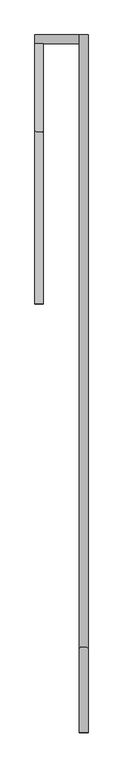
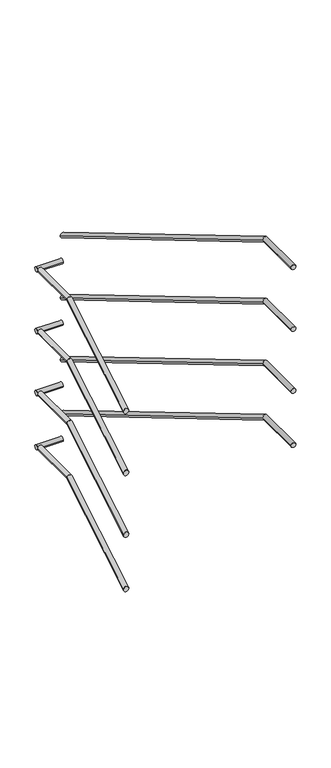
"""IFC4 building model written with IfcOpenShell, lengths in millimetres: railing geometry."""

from ifc_helpers import new_model, si_unit, frame, origin, place, context, project, spatial, circle_curve, ellipse_curve, source, transform, mapped, element, save
from ifc_brep_helpers import plane_surface, cylinder_surface, advanced_brep


def railing_415aae61(model_context):
    return source(origin(), model_context, "Body", "AdvancedBrep", [
        advanced_brep(
        [(52769.6, 14329.5208589, 10810.697424), (52799.6, 14329.5208589, 10810.697424), (52769.6, 14933.6395577, 11169.5073179), (52799.6, 14933.6395577, 11169.5073179), (52769.6, 15239.9208589, 11169.5073179), (52799.6, 15239.9208589, 11169.5073179)],
        [
            (0, 1, ellipse_curve(frame((52784.6, 14329.5208589, 10810.697424), z_axis=(0.0, -1.0, 0.0), x_axis=(0.0, 0.0, -1.0)), 17.4462575, 15.0)),
            (1, 0, ellipse_curve(frame((52784.6, 14329.5208589, 10810.697424), z_axis=(0.0, -1.0, 0.0), x_axis=(0.0, 0.0, -1.0)), 17.4462575, 15.0)),
            (0, 2),
            (2, 3, ellipse_curve(frame((52784.6, 14933.6395577, 11169.5073179), z_axis=(0.0, -0.9643088850075937, -0.26477986006381166), x_axis=(0.0, 0.2647798600638126, -0.9643088850075935)), 15.5551818, 15.0)),
            (3, 1),
            (3, 2, ellipse_curve(frame((52784.6, 14933.6395577, 11169.5073179), z_axis=(0.0, -0.9643088850075937, -0.26477986006381166), x_axis=(0.0, 0.2647798600638126, -0.9643088850075935)), 15.5551818, 15.0)),
            (4, 5, circle_curve(frame((52784.6, 15239.9208589, 11169.5073179), z_axis=(0.0, 1.0, 0.0), x_axis=(1.0, 0.0, 0.0)), 15.0)),
            (5, 4, circle_curve(frame((52784.6, 15239.9208589, 11169.5073179), z_axis=(0.0, 1.0, 0.0), x_axis=(1.0, 0.0, 0.0)), 15.0)),
            (2, 4),
            (5, 3),
        ],
        [
            plane_surface(frame((52784.6, 14329.5208589, 10828.1436815), z_axis=(0.0, -1.0, 0.0), x_axis=(0.0, 0.0, 1.0))),
            cylinder_surface(frame((52784.6, 14337.180746, 10815.2469328), z_axis=(0.0, -0.8597832514091767, -0.5106591432612018), x_axis=(1.0, 0.0, 0.0)), 15.0),
            plane_surface(frame((52784.6, 15239.9208589, 11184.5073179), z_axis=(0.0, 1.0, 0.0), x_axis=(0.0, 0.0, 1.0))),
            cylinder_surface(frame((52784.6, 14929.5208589, 11169.5073179), z_axis=(0.0, -1.0, 0.0), x_axis=(1.0, 0.0, 0.0)), 15.0),
        ],
        [
            (0, [[1, 2]]),
            (1, [[-1, 3, 4, 5]]),
            (1, [[-2, -5, 6, -3]]),
            (2, [[7, 8]]),
            (3, [[-4, 9, -8, 10]]),
            (3, [[-6, -10, -7, -9]]),
        ],
    ),
        advanced_brep(
        [(52769.6, 15269.9208589, 11169.5073179), (52769.6, 15239.9208589, 11169.5073179), (52925.4, 15269.9208589, 11169.5073179), (52925.4, 15239.9208589, 11169.5073179)],
        [
            (0, 1, circle_curve(frame((52769.6, 15254.9208589, 11169.5073179), z_axis=(-1.0, 0.0, 0.0), x_axis=(0.0, -1.0, 0.0)), 15.0)),
            (1, 0, circle_curve(frame((52769.6, 15254.9208589, 11169.5073179), z_axis=(-1.0, 0.0, 0.0), x_axis=(0.0, -1.0, 0.0)), 15.0)),
            (2, 3, circle_curve(frame((52925.4, 15254.9208589, 11169.5073179), z_axis=(1.0, 0.0, 0.0), x_axis=(0.0, -1.0, 0.0)), 15.0)),
            (3, 2, circle_curve(frame((52925.4, 15254.9208589, 11169.5073179), z_axis=(1.0, 0.0, 0.0), x_axis=(0.0, -1.0, 0.0)), 15.0)),
            (0, 2),
            (3, 1),
        ],
        [
            plane_surface(frame((52769.6, 15254.9208589, 11184.5073179), z_axis=(-1.0, 0.0, 0.0), x_axis=(0.0, 1.0, 0.0))),
            plane_surface(frame((52925.4, 15254.9208589, 11184.5073179), z_axis=(1.0, 0.0, 0.0), x_axis=(0.0, 1.0, 0.0))),
            cylinder_surface(frame((52769.6, 15254.9208589, 11169.5073179), z_axis=(-1.0, 0.0, 0.0), x_axis=(0.0, -1.0, 0.0)), 15.0),
        ],
        [
            (0, [[1, 2]]),
            (1, [[3, 4]]),
            (2, [[-1, 5, -4, 6]]),
            (2, [[-2, -6, -3, -5]]),
        ],
    ),
        advanced_brep(
        [(52955.4, 15269.9208589, 11321.2477271), (52925.4, 15269.9208589, 11321.2477271), (52955.4, 13125.40216, 12594.9618634), (52925.4, 13125.40216, 12594.9618634), (52955.4, 12829.5208589, 12594.9618634), (52925.4, 12829.5208589, 12594.9618634)],
        [
            (0, 1, ellipse_curve(frame((52940.4, 15269.9208589, 11321.2477271), z_axis=(0.0, 1.0, 0.0), x_axis=(0.0, 0.0, -1.0)), 17.4462575, 15.0)),
            (1, 0, ellipse_curve(frame((52940.4, 15269.9208589, 11321.2477271), z_axis=(0.0, 1.0, 0.0), x_axis=(0.0, 0.0, -1.0)), 17.4462575, 15.0)),
            (0, 2),
            (2, 3, ellipse_curve(frame((52940.4, 13125.40216, 12594.9618634), z_axis=(0.0, 0.9643088850075937, -0.26477986006381166), x_axis=(0.0, -0.2647798600638126, -0.9643088850075935)), 15.5551818, 15.0)),
            (3, 1),
            (3, 2, ellipse_curve(frame((52940.4, 13125.40216, 12594.9618634), z_axis=(0.0, 0.9643088850075937, -0.26477986006381166), x_axis=(0.0, -0.2647798600638126, -0.9643088850075935)), 15.5551818, 15.0)),
            (4, 5, circle_curve(frame((52940.4, 12829.5208589, 12594.9618634), z_axis=(0.0, -1.0, 0.0), x_axis=(-1.0, 0.0, 0.0)), 15.0)),
            (5, 4, circle_curve(frame((52940.4, 12829.5208589, 12594.9618634), z_axis=(0.0, -1.0, 0.0), x_axis=(-1.0, 0.0, 0.0)), 15.0)),
            (2, 4),
            (5, 3),
        ],
        [
            plane_surface(frame((52940.4, 15269.9208589, 11338.6939846), z_axis=(0.0, 1.0, 0.0), x_axis=(0.0, 0.0, -1.0))),
            cylinder_surface(frame((52940.4, 15262.2609717, 11325.7972358), z_axis=(0.0, 0.8597832514091767, -0.5106591432612018), x_axis=(-1.0, 0.0, 0.0)), 15.0),
            plane_surface(frame((52940.4, 12829.5208589, 12609.9618634), z_axis=(0.0, -1.0, 0.0), x_axis=(0.0, 0.0, -1.0))),
            cylinder_surface(frame((52940.4, 13129.5208589, 12594.9618634), z_axis=(0.0, 1.0, 0.0), x_axis=(-1.0, 0.0, 0.0)), 15.0),
        ],
        [
            (0, [[1, 2]]),
            (1, [[-1, 3, 4, 5]]),
            (1, [[-2, -5, 6, -3]]),
            (2, [[7, 8]]),
            (3, [[-4, 9, -8, 10]]),
            (3, [[-6, -10, -7, -9]]),
        ],
    ),
        advanced_brep(
        [(52769.6, 14329.5208589, 10010.697424), (52799.6, 14329.5208589, 10010.697424), (52769.6, 14933.6395577, 10369.5073179), (52799.6, 14933.6395577, 10369.5073179), (52769.6, 15239.9208589, 10369.5073179), (52799.6, 15239.9208589, 10369.5073179)],
        [
            (0, 1, ellipse_curve(frame((52784.6, 14329.5208589, 10010.697424), z_axis=(0.0, -1.0, 0.0), x_axis=(0.0, 0.0, -1.0)), 17.4462575, 15.0)),
            (1, 0, ellipse_curve(frame((52784.6, 14329.5208589, 10010.697424), z_axis=(0.0, -1.0, 0.0), x_axis=(0.0, 0.0, -1.0)), 17.4462575, 15.0)),
            (0, 2),
            (2, 3, ellipse_curve(frame((52784.6, 14933.6395577, 10369.5073179), z_axis=(0.0, -0.9643088850075937, -0.26477986006381166), x_axis=(0.0, 0.2647798600638126, -0.9643088850075935)), 15.5551818, 15.0)),
            (3, 1),
            (3, 2, ellipse_curve(frame((52784.6, 14933.6395577, 10369.5073179), z_axis=(0.0, -0.9643088850075937, -0.26477986006381166), x_axis=(0.0, 0.2647798600638126, -0.9643088850075935)), 15.5551818, 15.0)),
            (4, 5, circle_curve(frame((52784.6, 15239.9208589, 10369.5073179), z_axis=(0.0, 1.0, 0.0), x_axis=(1.0, 0.0, 0.0)), 15.0)),
            (5, 4, circle_curve(frame((52784.6, 15239.9208589, 10369.5073179), z_axis=(0.0, 1.0, 0.0), x_axis=(1.0, 0.0, 0.0)), 15.0)),
            (2, 4),
            (5, 3),
        ],
        [
            plane_surface(frame((52784.6, 14329.5208589, 10028.1436815), z_axis=(0.0, -1.0, 0.0), x_axis=(0.0, 0.0, 1.0))),
            cylinder_surface(frame((52784.6, 14337.180746, 10015.2469328), z_axis=(0.0, -0.8597832514091767, -0.5106591432612018), x_axis=(1.0, 0.0, 0.0)), 15.0),
            plane_surface(frame((52784.6, 15239.9208589, 10384.5073179), z_axis=(0.0, 1.0, 0.0), x_axis=(0.0, 0.0, 1.0))),
            cylinder_surface(frame((52784.6, 14929.5208589, 10369.5073179), z_axis=(0.0, -1.0, 0.0), x_axis=(1.0, 0.0, 0.0)), 15.0),
        ],
        [
            (0, [[1, 2]]),
            (1, [[-1, 3, 4, 5]]),
            (1, [[-2, -5, 6, -3]]),
            (2, [[7, 8]]),
            (3, [[-4, 9, -8, 10]]),
            (3, [[-6, -10, -7, -9]]),
        ],
    ),
        advanced_brep(
        [(52769.6, 15269.9208589, 10369.5073179), (52769.6, 15239.9208589, 10369.5073179), (52925.4, 15269.9208589, 10369.5073179), (52925.4, 15239.9208589, 10369.5073179)],
        [
            (0, 1, circle_curve(frame((52769.6, 15254.9208589, 10369.5073179), z_axis=(-1.0, 0.0, 0.0), x_axis=(0.0, -1.0, 0.0)), 15.0)),
            (1, 0, circle_curve(frame((52769.6, 15254.9208589, 10369.5073179), z_axis=(-1.0, 0.0, 0.0), x_axis=(0.0, -1.0, 0.0)), 15.0)),
            (2, 3, circle_curve(frame((52925.4, 15254.9208589, 10369.5073179), z_axis=(1.0, 0.0, 0.0), x_axis=(0.0, -1.0, 0.0)), 15.0)),
            (3, 2, circle_curve(frame((52925.4, 15254.9208589, 10369.5073179), z_axis=(1.0, 0.0, 0.0), x_axis=(0.0, -1.0, 0.0)), 15.0)),
            (0, 2),
            (3, 1),
        ],
        [
            plane_surface(frame((52769.6, 15254.9208589, 10384.5073179), z_axis=(-1.0, 0.0, 0.0), x_axis=(0.0, 1.0, 0.0))),
            plane_surface(frame((52925.4, 15254.9208589, 10384.5073179), z_axis=(1.0, 0.0, 0.0), x_axis=(0.0, 1.0, 0.0))),
            cylinder_surface(frame((52769.6, 15254.9208589, 10369.5073179), z_axis=(-1.0, 0.0, 0.0), x_axis=(0.0, -1.0, 0.0)), 15.0),
        ],
        [
            (0, [[1, 2]]),
            (1, [[3, 4]]),
            (2, [[-1, 5, -4, 6]]),
            (2, [[-2, -6, -3, -5]]),
        ],
    ),
        advanced_brep(
        [(52955.4, 15269.9208589, 10521.2477271), (52925.4, 15269.9208589, 10521.2477271), (52955.4, 13125.40216, 11794.9618634), (52925.4, 13125.40216, 11794.9618634), (52955.4, 12829.5208589, 11794.9618634), (52925.4, 12829.5208589, 11794.9618634)],
        [
            (0, 1, ellipse_curve(frame((52940.4, 15269.9208589, 10521.2477271), z_axis=(0.0, 1.0, 0.0), x_axis=(0.0, 0.0, -1.0)), 17.4462575, 15.0)),
            (1, 0, ellipse_curve(frame((52940.4, 15269.9208589, 10521.2477271), z_axis=(0.0, 1.0, 0.0), x_axis=(0.0, 0.0, -1.0)), 17.4462575, 15.0)),
            (0, 2),
            (2, 3, ellipse_curve(frame((52940.4, 13125.40216, 11794.9618634), z_axis=(0.0, 0.9643088850075937, -0.26477986006381166), x_axis=(0.0, -0.2647798600638126, -0.9643088850075935)), 15.5551818, 15.0)),
            (3, 1),
            (3, 2, ellipse_curve(frame((52940.4, 13125.40216, 11794.9618634), z_axis=(0.0, 0.9643088850075937, -0.26477986006381166), x_axis=(0.0, -0.2647798600638126, -0.9643088850075935)), 15.5551818, 15.0)),
            (4, 5, circle_curve(frame((52940.4, 12829.5208589, 11794.9618634), z_axis=(0.0, -1.0, 0.0), x_axis=(-1.0, 0.0, 0.0)), 15.0)),
            (5, 4, circle_curve(frame((52940.4, 12829.5208589, 11794.9618634), z_axis=(0.0, -1.0, 0.0), x_axis=(-1.0, 0.0, 0.0)), 15.0)),
            (2, 4),
            (5, 3),
        ],
        [
            plane_surface(frame((52940.4, 15269.9208589, 10538.6939846), z_axis=(0.0, 1.0, 0.0), x_axis=(0.0, 0.0, -1.0))),
            cylinder_surface(frame((52940.4, 15262.2609717, 10525.7972358), z_axis=(0.0, 0.8597832514091767, -0.5106591432612018), x_axis=(-1.0, 0.0, 0.0)), 15.0),
            plane_surface(frame((52940.4, 12829.5208589, 11809.9618634), z_axis=(0.0, -1.0, 0.0), x_axis=(0.0, 0.0, -1.0))),
            cylinder_surface(frame((52940.4, 13129.5208589, 11794.9618634), z_axis=(0.0, 1.0, 0.0), x_axis=(-1.0, 0.0, 0.0)), 15.0),
        ],
        [
            (0, [[1, 2]]),
            (1, [[-1, 3, 4, 5]]),
            (1, [[-2, -5, 6, -3]]),
            (2, [[7, 8]]),
            (3, [[-4, 9, -8, 10]]),
            (3, [[-6, -10, -7, -9]]),
        ],
    ),
        advanced_brep(
        [(52769.6, 14329.5208589, 10410.697424), (52799.6, 14329.5208589, 10410.697424), (52769.6, 14933.6395577, 10769.5073179), (52799.6, 14933.6395577, 10769.5073179), (52769.6, 15239.9208589, 10769.5073179), (52799.6, 15239.9208589, 10769.5073179)],
        [
            (0, 1, ellipse_curve(frame((52784.6, 14329.5208589, 10410.697424), z_axis=(0.0, -1.0, 0.0), x_axis=(0.0, 0.0, -1.0)), 17.4462575, 15.0)),
            (1, 0, ellipse_curve(frame((52784.6, 14329.5208589, 10410.697424), z_axis=(0.0, -1.0, 0.0), x_axis=(0.0, 0.0, -1.0)), 17.4462575, 15.0)),
            (0, 2),
            (2, 3, ellipse_curve(frame((52784.6, 14933.6395577, 10769.5073179), z_axis=(0.0, -0.9643088850075937, -0.26477986006381166), x_axis=(0.0, 0.2647798600638126, -0.9643088850075935)), 15.5551818, 15.0)),
            (3, 1),
            (3, 2, ellipse_curve(frame((52784.6, 14933.6395577, 10769.5073179), z_axis=(0.0, -0.9643088850075937, -0.26477986006381166), x_axis=(0.0, 0.2647798600638126, -0.9643088850075935)), 15.5551818, 15.0)),
            (4, 5, circle_curve(frame((52784.6, 15239.9208589, 10769.5073179), z_axis=(0.0, 1.0, 0.0), x_axis=(1.0, 0.0, 0.0)), 15.0)),
            (5, 4, circle_curve(frame((52784.6, 15239.9208589, 10769.5073179), z_axis=(0.0, 1.0, 0.0), x_axis=(1.0, 0.0, 0.0)), 15.0)),
            (2, 4),
            (5, 3),
        ],
        [
            plane_surface(frame((52784.6, 14329.5208589, 10428.1436815), z_axis=(0.0, -1.0, 0.0), x_axis=(0.0, 0.0, 1.0))),
            cylinder_surface(frame((52784.6, 14337.180746, 10415.2469328), z_axis=(0.0, -0.8597832514091767, -0.5106591432612018), x_axis=(1.0, 0.0, 0.0)), 15.0),
            plane_surface(frame((52784.6, 15239.9208589, 10784.5073179), z_axis=(0.0, 1.0, 0.0), x_axis=(0.0, 0.0, 1.0))),
            cylinder_surface(frame((52784.6, 14929.5208589, 10769.5073179), z_axis=(0.0, -1.0, 0.0), x_axis=(1.0, 0.0, 0.0)), 15.0),
        ],
        [
            (0, [[1, 2]]),
            (1, [[-1, 3, 4, 5]]),
            (1, [[-2, -5, 6, -3]]),
            (2, [[7, 8]]),
            (3, [[-4, 9, -8, 10]]),
            (3, [[-6, -10, -7, -9]]),
        ],
    ),
        advanced_brep(
        [(52769.6, 15269.9208589, 10769.5073179), (52769.6, 15239.9208589, 10769.5073179), (52925.4, 15269.9208589, 10769.5073179), (52925.4, 15239.9208589, 10769.5073179)],
        [
            (0, 1, circle_curve(frame((52769.6, 15254.9208589, 10769.5073179), z_axis=(-1.0, 0.0, 0.0), x_axis=(0.0, -1.0, 0.0)), 15.0)),
            (1, 0, circle_curve(frame((52769.6, 15254.9208589, 10769.5073179), z_axis=(-1.0, 0.0, 0.0), x_axis=(0.0, -1.0, 0.0)), 15.0)),
            (2, 3, circle_curve(frame((52925.4, 15254.9208589, 10769.5073179), z_axis=(1.0, 0.0, 0.0), x_axis=(0.0, -1.0, 0.0)), 15.0)),
            (3, 2, circle_curve(frame((52925.4, 15254.9208589, 10769.5073179), z_axis=(1.0, 0.0, 0.0), x_axis=(0.0, -1.0, 0.0)), 15.0)),
            (0, 2),
            (3, 1),
        ],
        [
            plane_surface(frame((52769.6, 15254.9208589, 10784.5073179), z_axis=(-1.0, 0.0, 0.0), x_axis=(0.0, 1.0, 0.0))),
            plane_surface(frame((52925.4, 15254.9208589, 10784.5073179), z_axis=(1.0, 0.0, 0.0), x_axis=(0.0, 1.0, 0.0))),
            cylinder_surface(frame((52769.6, 15254.9208589, 10769.5073179), z_axis=(-1.0, 0.0, 0.0), x_axis=(0.0, -1.0, 0.0)), 15.0),
        ],
        [
            (0, [[1, 2]]),
            (1, [[3, 4]]),
            (2, [[-1, 5, -4, 6]]),
            (2, [[-2, -6, -3, -5]]),
        ],
    ),
        advanced_brep(
        [(52955.4, 15269.9208589, 10921.2477271), (52925.4, 15269.9208589, 10921.2477271), (52955.4, 13125.40216, 12194.9618634), (52925.4, 13125.40216, 12194.9618634), (52955.4, 12829.5208589, 12194.9618634), (52925.4, 12829.5208589, 12194.9618634)],
        [
            (0, 1, ellipse_curve(frame((52940.4, 15269.9208589, 10921.2477271), z_axis=(0.0, 1.0, 0.0), x_axis=(0.0, 0.0, -1.0)), 17.4462575, 15.0)),
            (1, 0, ellipse_curve(frame((52940.4, 15269.9208589, 10921.2477271), z_axis=(0.0, 1.0, 0.0), x_axis=(0.0, 0.0, -1.0)), 17.4462575, 15.0)),
            (0, 2),
            (2, 3, ellipse_curve(frame((52940.4, 13125.40216, 12194.9618634), z_axis=(0.0, 0.9643088850075937, -0.26477986006381166), x_axis=(0.0, -0.2647798600638126, -0.9643088850075935)), 15.5551818, 15.0)),
            (3, 1),
            (3, 2, ellipse_curve(frame((52940.4, 13125.40216, 12194.9618634), z_axis=(0.0, 0.9643088850075937, -0.26477986006381166), x_axis=(0.0, -0.2647798600638126, -0.9643088850075935)), 15.5551818, 15.0)),
            (4, 5, circle_curve(frame((52940.4, 12829.5208589, 12194.9618634), z_axis=(0.0, -1.0, 0.0), x_axis=(-1.0, 0.0, 0.0)), 15.0)),
            (5, 4, circle_curve(frame((52940.4, 12829.5208589, 12194.9618634), z_axis=(0.0, -1.0, 0.0), x_axis=(-1.0, 0.0, 0.0)), 15.0)),
            (2, 4),
            (5, 3),
        ],
        [
            plane_surface(frame((52940.4, 15269.9208589, 10938.6939846), z_axis=(0.0, 1.0, 0.0), x_axis=(0.0, 0.0, -1.0))),
            cylinder_surface(frame((52940.4, 15262.2609717, 10925.7972358), z_axis=(0.0, 0.8597832514091767, -0.5106591432612018), x_axis=(-1.0, 0.0, 0.0)), 15.0),
            plane_surface(frame((52940.4, 12829.5208589, 12209.9618634), z_axis=(0.0, -1.0, 0.0), x_axis=(0.0, 0.0, -1.0))),
            cylinder_surface(frame((52940.4, 13129.5208589, 12194.9618634), z_axis=(0.0, 1.0, 0.0), x_axis=(-1.0, 0.0, 0.0)), 15.0),
        ],
        [
            (0, [[1, 2]]),
            (1, [[-1, 3, 4, 5]]),
            (1, [[-2, -5, 6, -3]]),
            (2, [[7, 8]]),
            (3, [[-4, 9, -8, 10]]),
            (3, [[-6, -10, -7, -9]]),
        ],
    ),
        advanced_brep(
        [(52769.6, 14329.5208589, 9660.697424), (52799.6, 14329.5208589, 9660.697424), (52769.6, 14933.6395577, 10019.5073179), (52799.6, 14933.6395577, 10019.5073179), (52769.6, 15239.9208589, 10019.5073179), (52799.6, 15239.9208589, 10019.5073179)],
        [
            (0, 1, ellipse_curve(frame((52784.6, 14329.5208589, 9660.697424), z_axis=(0.0, -1.0, 0.0), x_axis=(0.0, 0.0, -1.0)), 17.4462575, 15.0)),
            (1, 0, ellipse_curve(frame((52784.6, 14329.5208589, 9660.697424), z_axis=(0.0, -1.0, 0.0), x_axis=(0.0, 0.0, -1.0)), 17.4462575, 15.0)),
            (0, 2),
            (2, 3, ellipse_curve(frame((52784.6, 14933.6395577, 10019.5073179), z_axis=(0.0, -0.9643088850075937, -0.26477986006381166), x_axis=(0.0, 0.2647798600638126, -0.9643088850075935)), 15.5551818, 15.0)),
            (3, 1),
            (3, 2, ellipse_curve(frame((52784.6, 14933.6395577, 10019.5073179), z_axis=(0.0, -0.9643088850075937, -0.26477986006381166), x_axis=(0.0, 0.2647798600638126, -0.9643088850075935)), 15.5551818, 15.0)),
            (4, 5, circle_curve(frame((52784.6, 15239.9208589, 10019.5073179), z_axis=(0.0, 1.0, 0.0), x_axis=(1.0, 0.0, 0.0)), 15.0)),
            (5, 4, circle_curve(frame((52784.6, 15239.9208589, 10019.5073179), z_axis=(0.0, 1.0, 0.0), x_axis=(1.0, 0.0, 0.0)), 15.0)),
            (2, 4),
            (5, 3),
        ],
        [
            plane_surface(frame((52784.6, 14329.5208589, 9678.1436815), z_axis=(0.0, -1.0, 0.0), x_axis=(0.0, 0.0, 1.0))),
            cylinder_surface(frame((52784.6, 14337.180746, 9665.2469328), z_axis=(0.0, -0.8597832514091767, -0.5106591432612018), x_axis=(1.0, 0.0, 0.0)), 15.0),
            plane_surface(frame((52784.6, 15239.9208589, 10034.5073179), z_axis=(0.0, 1.0, 0.0), x_axis=(0.0, 0.0, 1.0))),
            cylinder_surface(frame((52784.6, 14929.5208589, 10019.5073179), z_axis=(0.0, -1.0, 0.0), x_axis=(1.0, 0.0, 0.0)), 15.0),
        ],
        [
            (0, [[1, 2]]),
            (1, [[-1, 3, 4, 5]]),
            (1, [[-2, -5, 6, -3]]),
            (2, [[7, 8]]),
            (3, [[-4, 9, -8, 10]]),
            (3, [[-6, -10, -7, -9]]),
        ],
    ),
        advanced_brep(
        [(52769.6, 15269.9208589, 10019.5073179), (52769.6, 15239.9208589, 10019.5073179), (52925.4, 15269.9208589, 10019.5073179), (52925.4, 15239.9208589, 10019.5073179)],
        [
            (0, 1, circle_curve(frame((52769.6, 15254.9208589, 10019.5073179), z_axis=(-1.0, 0.0, 0.0), x_axis=(0.0, -1.0, 0.0)), 15.0)),
            (1, 0, circle_curve(frame((52769.6, 15254.9208589, 10019.5073179), z_axis=(-1.0, 0.0, 0.0), x_axis=(0.0, -1.0, 0.0)), 15.0)),
            (2, 3, circle_curve(frame((52925.4, 15254.9208589, 10019.5073179), z_axis=(1.0, 0.0, 0.0), x_axis=(0.0, -1.0, 0.0)), 15.0)),
            (3, 2, circle_curve(frame((52925.4, 15254.9208589, 10019.5073179), z_axis=(1.0, 0.0, 0.0), x_axis=(0.0, -1.0, 0.0)), 15.0)),
            (0, 2),
            (3, 1),
        ],
        [
            plane_surface(frame((52769.6, 15254.9208589, 10034.5073179), z_axis=(-1.0, 0.0, 0.0), x_axis=(0.0, 1.0, 0.0))),
            plane_surface(frame((52925.4, 15254.9208589, 10034.5073179), z_axis=(1.0, 0.0, 0.0), x_axis=(0.0, 1.0, 0.0))),
            cylinder_surface(frame((52769.6, 15254.9208589, 10019.5073179), z_axis=(-1.0, 0.0, 0.0), x_axis=(0.0, -1.0, 0.0)), 15.0),
        ],
        [
            (0, [[1, 2]]),
            (1, [[3, 4]]),
            (2, [[-1, 5, -4, 6]]),
            (2, [[-2, -6, -3, -5]]),
        ],
    ),
        advanced_brep(
        [(52955.4, 15269.9208589, 10171.2477271), (52925.4, 15269.9208589, 10171.2477271), (52955.4, 13125.40216, 11444.9618634), (52925.4, 13125.40216, 11444.9618634), (52955.4, 12829.5208589, 11444.9618634), (52925.4, 12829.5208589, 11444.9618634)],
        [
            (0, 1, ellipse_curve(frame((52940.4, 15269.9208589, 10171.2477271), z_axis=(0.0, 1.0, 0.0), x_axis=(0.0, 0.0, -1.0)), 17.4462575, 15.0)),
            (1, 0, ellipse_curve(frame((52940.4, 15269.9208589, 10171.2477271), z_axis=(0.0, 1.0, 0.0), x_axis=(0.0, 0.0, -1.0)), 17.4462575, 15.0)),
            (0, 2),
            (2, 3, ellipse_curve(frame((52940.4, 13125.40216, 11444.9618634), z_axis=(0.0, 0.9643088850075937, -0.26477986006381166), x_axis=(0.0, -0.2647798600638126, -0.9643088850075935)), 15.5551818, 15.0)),
            (3, 1),
            (3, 2, ellipse_curve(frame((52940.4, 13125.40216, 11444.9618634), z_axis=(0.0, 0.9643088850075937, -0.26477986006381166), x_axis=(0.0, -0.2647798600638126, -0.9643088850075935)), 15.5551818, 15.0)),
            (4, 5, circle_curve(frame((52940.4, 12829.5208589, 11444.9618634), z_axis=(0.0, -1.0, 0.0), x_axis=(-1.0, 0.0, 0.0)), 15.0)),
            (5, 4, circle_curve(frame((52940.4, 12829.5208589, 11444.9618634), z_axis=(0.0, -1.0, 0.0), x_axis=(-1.0, 0.0, 0.0)), 15.0)),
            (2, 4),
            (5, 3),
        ],
        [
            plane_surface(frame((52940.4, 15269.9208589, 10188.6939846), z_axis=(0.0, 1.0, 0.0), x_axis=(0.0, 0.0, -1.0))),
            cylinder_surface(frame((52940.4, 15262.2609717, 10175.7972358), z_axis=(0.0, 0.8597832514091767, -0.5106591432612018), x_axis=(-1.0, 0.0, 0.0)), 15.0),
            plane_surface(frame((52940.4, 12829.5208589, 11459.9618634), z_axis=(0.0, -1.0, 0.0), x_axis=(0.0, 0.0, -1.0))),
            cylinder_surface(frame((52940.4, 13129.5208589, 11444.9618634), z_axis=(0.0, 1.0, 0.0), x_axis=(-1.0, 0.0, 0.0)), 15.0),
        ],
        [
            (0, [[1, 2]]),
            (1, [[-1, 3, 4, 5]]),
            (1, [[-2, -5, 6, -3]]),
            (2, [[7, 8]]),
            (3, [[-4, 9, -8, 10]]),
            (3, [[-6, -10, -7, -9]]),
        ],
    ),
    ])


if __name__ == "__main__":
    model = new_model("IFC4")
    model_context = context("Model", 3, world=origin())
    ifc_project = project(units=[si_unit("LENGTHUNIT", "METRE", prefix="MILLI")], contexts=[model_context])
    site = spatial("IfcSite", under=ifc_project)
    building = spatial("IfcBuilding", under=site)
    placement = place(None, origin())
    railing_shape = railing_415aae61(model_context)
    element("IfcRailing", 1, at=placement, inside=building, context=model_context, shape_type="MappedRepresentation", body=[
        mapped(railing_shape, transform((0.0, 0.0, 0.0), x_axis=(1.0, 0.0, 0.0), y_axis=(0.0, 1.0, 0.0), z_axis=(0.0, 0.0, 1.0))),
    ])
    save(model, "model.ifc")
